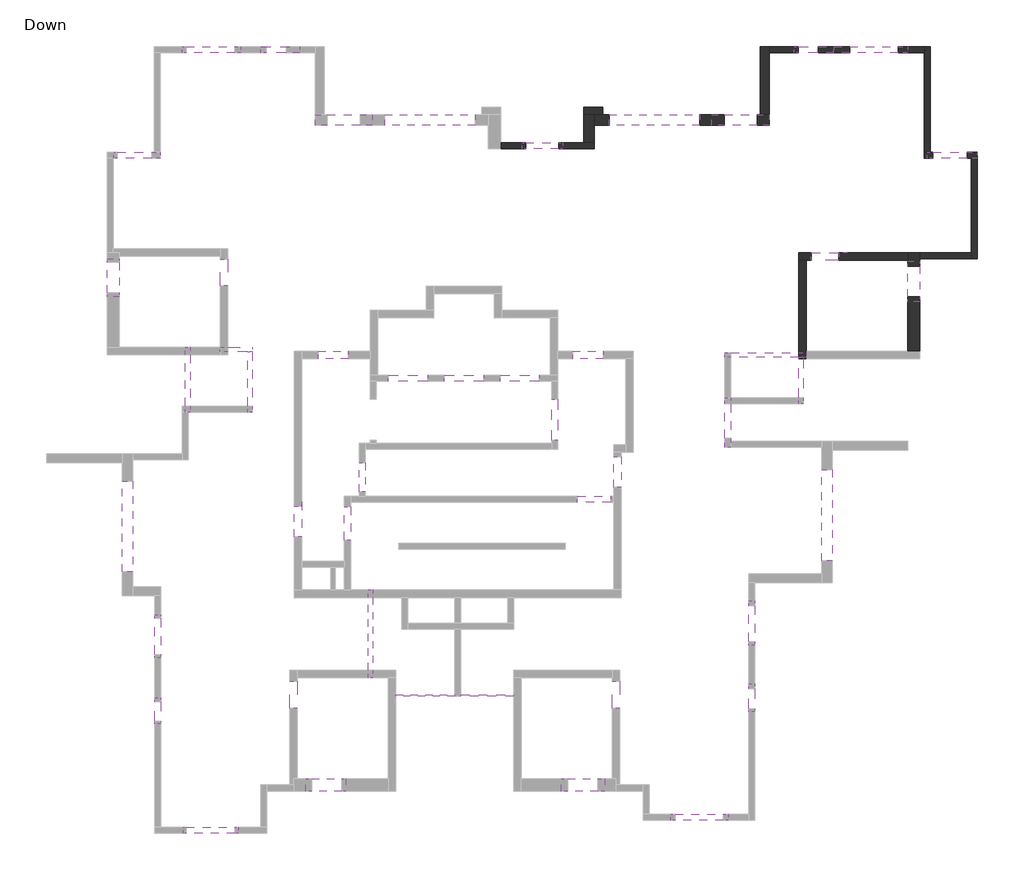
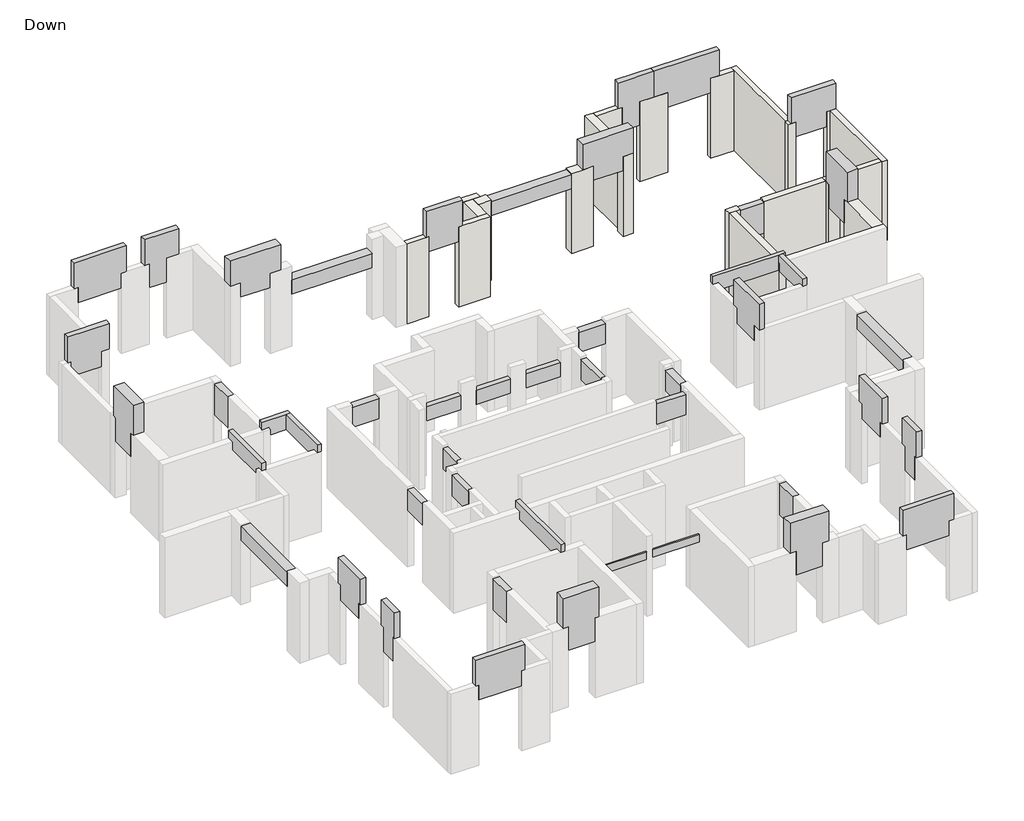
# One storey, part 3 of 3: 47 beams, 21 walls.
"""IFC4 building model written with IfcOpenShell, lengths in millimetres."""

from ifc_helpers import new_model, si_unit, frame, origin, place, context, project, spatial, polyline, outline, extrude, faceted_brep, element, save

model = new_model("IFC4")

# Units and contexts
model_context = context("Model", 3, world=origin())
ifc_project = project(units=[si_unit("LENGTHUNIT", "METRE", prefix="MILLI")], contexts=[model_context])

# Site, building, storey
site = spatial("IfcSite", under=ifc_project)
building = spatial("IfcBuilding", under=site)
storey = spatial("IfcBuildingStorey", under=building, Name="Down", Elevation=0.0)

# Beams
placement = place(None, origin())
element("IfcBeam", 1, ObjectType="Concrete Rectengular Beam : 15/60", at=placement, inside=storey, context=model_context, shape_type="Brep", body=[
    faceted_brep([(-3745.4992849, -160.4554551, 3450.0), (-3745.4992849, -10.4554551, 3450.0), (-6449.3881109, -10.4554551, 3450.0), (-6449.3881109, -160.4554551, 3450.0), (-3995.4992849, -160.4554551, 3450.0), (-3845.4992849, -160.4554551, 3450.0), (-6449.3881109, -160.4554551, 3150.0), (-6249.3881109, -160.4554551, 3150.0), (-6249.3881109, -160.4554551, 2850.0), (-3995.4992849, -160.4554551, 2850.0), (-3995.4992849, -160.4554551, 3150.0), (-3845.4992849, -160.4554551, 3150.0), (-3745.4992849, -160.4554551, 3150.0), (-3995.4992849, -10.4554551, 2850.0), (-6249.3881109, -10.4554551, 2850.0), (-3745.4992849, -10.4554551, 3150.0), (-3995.4992849, -10.4554551, 3150.0), (-3995.4992849, -10.4554551, 2950.0), (-6249.3881109, -10.4554551, 3150.0), (-6449.3881109, -10.4554551, 3150.0)], [[[0, 1, 2, 3, 4, 5]], [[0, 5, 4, 3, 6, 7, 8, 9, 10, 11, 12]], [[13, 9, 8, 14]], [[2, 1, 15, 16, 17, 13, 14, 18, 19]], [[1, 0, 12, 15]], [[3, 2, 19, 6]], [[16, 10, 9, 13, 17]], [[10, 16, 15, 12, 11]], [[7, 18, 14, 8]], [[18, 7, 6, 19]]]),
])
element("IfcBeam", 2, ObjectType="Concrete Rectengular Beam : 15/60", at=placement, inside=storey, context=model_context, shape_type="SweptSolid", body=[
    extrude(outline(polyline([(-1713.3876412, 3450.0), (-160.4554551, 3450.0), (-160.4554551, 3150.0), (-210.9535871, 3150.0), (-210.9535871, 2850.0), (-1513.3876412, 2850.0), (-1513.3876412, 3150.0), (-1713.3876412, 3150.0), (-1713.3876412, 3450.0)])), frame((-3995.4992849, 0.0, 0.0), z_axis=(1.0, 0.0, 0.0), x_axis=(0.0, 1.0, 0.0)), (0.0, 0.0, 1.0), 150.0),
])
element("IfcBeam", 3, ObjectType="Concrete Rectengular Beam : 15/60", at=placement, inside=storey, context=model_context, shape_type="Brep", body=[
    faceted_brep([(-23152.2127458, 170.2815538, 3450.0), (-23152.2127458, 20.2815538, 3450.0), (-22250.9487358, 20.2815538, 3450.0), (-22100.9487358, 20.2815538, 3450.0), (-22100.9487358, 170.2815538, 3450.0), (-23152.2127458, 20.2815538, 3150.0), (-22902.2127458, 20.2815538, 3150.0), (-22902.2127458, 20.2815538, 2850.0), (-22250.9487358, 20.2815538, 2850.0), (-22100.9487358, 20.2815538, 2850.0), (-22100.9487358, 20.2815538, 2950.0), (-22100.9487358, 20.2815538, 3150.0), (-22100.9487358, 170.2815538, 2850.0), (-22902.2127458, 170.2815538, 2850.0), (-22100.9487358, 170.2815538, 3150.0), (-22100.9487358, 170.2815538, 2950.0), (-22902.2127458, 170.2815538, 2950.0), (-22902.2127458, 170.2815538, 3150.0), (-23152.2127458, 170.2815538, 3150.0)], [[[0, 1, 2, 3, 4]], [[3, 2, 1, 5, 6, 7, 8, 9, 10, 11]], [[12, 9, 8, 7, 13]], [[0, 4, 14, 15, 12, 13, 16, 17, 18]], [[1, 0, 18, 5]], [[4, 3, 11, 10, 9, 12, 15, 14]], [[6, 17, 16, 13, 7]], [[17, 6, 5, 18]]]),
])
element("IfcBeam", 4, ObjectType="Concrete Rectengular Beam : 15/60", at=placement, inside=storey, context=model_context, shape_type="Brep", body=[
    faceted_brep([(-22250.9487358, -1984.190313, 3450.0), (-22100.9487358, -1984.190313, 3450.0), (-22100.9487358, 20.2815538, 3450.0), (-22250.9487358, 20.2815538, 3450.0), (-22250.9487358, 20.2815538, 2850.0), (-22250.9487358, -1784.190313, 2850.0), (-22250.9487358, -1784.190313, 3150.0), (-22250.9487358, -1984.190313, 3150.0), (-22100.9487358, 20.2815538, 2850.0), (-22100.9487358, -1784.190313, 2850.0), (-22100.9487358, -1984.190313, 3150.0), (-22100.9487358, -1784.190313, 3150.0), (-22100.9487358, 20.2815538, 2950.0), (-22100.9487358, 20.2815538, 3150.0)], [[[0, 1, 2, 3]], [[3, 4, 5, 6, 7, 0]], [[4, 8, 9, 5]], [[2, 1, 10, 11, 9, 8, 12, 13]], [[1, 0, 7, 10]], [[3, 2, 13, 12, 8, 4]], [[11, 6, 5, 9]], [[6, 11, 10, 7]]]),
])
element("IfcBeam", 5, ObjectType="Concrete Rectengular Beam : 15/60", at=placement, inside=storey, context=model_context, shape_type="SweptSolid", body=[
    extrude(outline(polyline([(-1984.190313, 3450.0), (170.2815538, 3450.0), (170.2815538, 3150.0), (-79.7184462, 3150.0), (-79.7184462, 2850.0), (-1784.190313, 2850.0), (-1784.190313, 3150.0), (-1984.190313, 3150.0), (-1984.190313, 3450.0)])), frame((-24310.0622873, 0.0, 0.0), z_axis=(1.0, 0.0, 0.0), x_axis=(0.0, 1.0, 0.0)), (0.0, 0.0, 1.0), 150.0),
])
element("IfcBeam", 6, ObjectType="Concrete Rectengular Beam : 15/60", at=placement, inside=storey, context=model_context, shape_type="Brep", body=[
    faceted_brep([(-18253.1541021, -10778.5353827, 3450.0), (-18103.1541021, -10778.5353827, 3450.0), (-18103.1541021, -7874.1201217, 3450.0), (-18253.1541021, -7874.1201217, 3450.0), (-18103.1541021, -10778.5353827, 3150.0), (-18103.1541021, -10528.5353827, 3150.0), (-18103.1541021, -10528.5353827, 3000.0), (-18103.1541021, -10528.5353827, 2850.0), (-18103.1541021, -8124.1201217, 2850.0), (-18103.1541021, -8124.1201217, 3000.0), (-18103.1541021, -8124.1201217, 3150.0), (-18103.1541021, -7874.1201217, 3150.0), (-18253.1541021, -10528.5353827, 2850.0), (-18253.1541021, -8124.1201217, 2850.0), (-18253.1541021, -7874.1201217, 3150.0), (-18253.1541021, -8124.1201217, 3150.0), (-18253.1541021, -8124.1201217, 2950.0), (-18253.1541021, -10528.5353827, 2950.0), (-18253.1541021, -10528.5353827, 3150.0), (-18253.1541021, -10778.5353827, 3150.0)], [[[0, 1, 2, 3]], [[2, 1, 4, 5, 6, 7, 8, 9, 10, 11]], [[7, 12, 13, 8]], [[0, 3, 14, 15, 16, 13, 12, 17, 18, 19]], [[1, 0, 19, 4]], [[3, 2, 11, 14]], [[5, 18, 17, 12, 7, 6]], [[18, 5, 4, 19]], [[15, 10, 9, 8, 13, 16]], [[10, 15, 14, 11]]]),
])
element("IfcBeam", 7, ObjectType="Concrete Rectengular Beam : 20/160", at=placement, inside=storey, context=model_context, shape_type="SweptSolid", body=[
    extrude(outline(polyline([(4170.0, -25146.2068588), (4170.0, -26693.7048776), (3150.0, -26693.7048776), (3150.0, -26578.3590155), (2570.0, -26578.3590155), (2570.0, -25426.4061116), (3150.0, -25426.4061116), (3150.0, -25146.2068588), (4170.0, -25146.2068588)])), frame((0.0, 6420.0664514, 0.0), z_axis=(0.0, 1.0, 0.0), x_axis=(0.0, 0.0, 1.0)), (0.0, 0.0, 1.0), 200.0),
])
element("IfcBeam", 8, ObjectType="Concrete Rectengular Beam : 20/160", at=placement, inside=storey, context=model_context, shape_type="SweptSolid", body=[
    extrude(outline(polyline([(4170.0, -22484.8686951), (4170.0, -24424.8686951), (3150.0, -24424.8686951), (3150.0, -24284.8686951), (2570.0, -24284.8686951), (2570.0, -22681.9251878), (3150.0, -22681.9251878), (3150.0, -22484.8686951), (4170.0, -22484.8686951)])), frame((0.0, 9925.9195024, 0.0), z_axis=(0.0, 1.0, 0.0), x_axis=(0.0, 0.0, 1.0)), (0.0, 0.0, 1.0), 200.0),
])
element("IfcBeam", 9, ObjectType="Concrete Rectengular Beam : 20/160", at=placement, inside=storey, context=model_context, shape_type="SweptSolid", body=[
    extrude(outline(polyline([(4170.0, -11807.2982207), (4170.0, -13147.2982207), (3150.0, -13147.2982207), (3150.0, -13043.4331692), (2570.0, -13043.4331692), (2570.0, -11941.4746047), (3150.0, -11941.4746047), (3150.0, -11807.2982207), (4170.0, -11807.2982207)])), frame((0.0, 6745.5504319, 0.0), z_axis=(0.0, 1.0, 0.0), x_axis=(0.0, 0.0, 1.0)), (0.0, 0.0, 1.0), 200.0),
])
element("IfcBeam", 10, ObjectType="Concrete Rectengular Beam : 20/160", at=placement, inside=storey, context=model_context, shape_type="SweptSolid", body=[
    extrude(outline(polyline([(4170.0, -388.4439243), (4170.0, -2828.4439243), (3150.0, -2828.4439243), (3150.0, -2302.4618118), (2570.0, -2302.4618118), (2570.0, -700.0390789), (3150.0, -700.0390789), (3150.0, -388.4439243), (4170.0, -388.4439243)])), frame((0.0, 9926.4176344, 0.0), z_axis=(0.0, 1.0, 0.0), x_axis=(0.0, 0.0, 1.0)), (0.0, 0.0, 1.0), 200.0),
])
element("IfcBeam", 11, ObjectType="Concrete Rectengular Beam : 20/160", at=placement, inside=storey, context=model_context, shape_type="SweptSolid", body=[
    extrude(outline(polyline([(4170.0, 1924.6637401), (4170.0, 261.8198592), (3150.0, 261.8198592), (3150.0, 442.019112), (2570.0, 442.019112), (2570.0, 1593.9720159), (3150.0, 1593.9720159), (3150.0, 1924.6637401), (4170.0, 1924.6637401)])), frame((0.0, 6420.0664514, 0.0), z_axis=(0.0, 1.0, 0.0), x_axis=(0.0, 0.0, 1.0)), (0.0, 0.0, 1.0), 200.0),
])
element("IfcBeam", 12, ObjectType="Concrete Rectengular Beam : 20/160", at=placement, inside=storey, context=model_context, shape_type="SweptSolid", body=[
    extrude(outline(polyline([(-3145.5397979, 4170.0), (-1513.3876412, 4170.0), (-1513.3876412, 3150.0), (-1713.3876412, 3150.0), (-1713.3876412, 2570.0), (-2845.5511191, 2570.0), (-2845.5511191, 3150.0), (-3145.5397979, 3150.0), (-3145.5397979, 4170.0)])), frame((-6449.3881109, 0.0, 0.0), z_axis=(1.0, 0.0, 0.0), x_axis=(0.0, 1.0, 0.0)), (0.0, 0.0, 1.0), 200.0),
])
element("IfcBeam", 13, ObjectType="Concrete Rectengular Beam : 20/160", at=placement, inside=storey, context=model_context, shape_type="SweptSolid", body=[
    extrude(outline(polyline([(-9711.6622931, 4170.0), (-8231.6622931, 4170.0), (-8231.6622931, 3150.0), (-8389.7150498, 3150.0), (-8389.7150498, 2570.0), (-9591.6622931, 2570.0), (-9591.6622931, 3150.0), (-9711.6622931, 3150.0), (-9711.6622931, 4170.0)])), frame((-5648.4371316, 0.0, 0.0), z_axis=(1.0, 0.0, 0.0), x_axis=(0.0, 1.0, 0.0)), (0.0, 0.0, 1.0), 200.0),
])
element("IfcBeam", 14, ObjectType="Concrete Rectengular Beam : 20/160", at=placement, inside=storey, context=model_context, shape_type="SweptSolid", body=[
    extrude(outline(polyline([(4170.0, -6333.7920507), (4170.0, -8233.7920507), (3150.0, -8233.7920507), (3150.0, -8093.7920507), (2570.0, -8093.7920507), (2570.0, -6499.9032247), (3150.0, -6499.9032247), (3150.0, -6333.7920507), (4170.0, -6333.7920507)])), frame((0.0, -15507.4032645, 0.0), z_axis=(0.0, 1.0, 0.0), x_axis=(0.0, 0.0, 1.0)), (0.0, 0.0, 1.0), 200.0),
])
element("IfcBeam", 15, ObjectType="Concrete Rectengular Beam : 20/160", at=placement, inside=storey, context=model_context, shape_type="SweptSolid", body=[
    extrude(outline(polyline([(4170.0, -22565.2739934), (4170.0, -24385.2739934), (3150.0, -24385.2739934), (3150.0, -24279.6609514), (2570.0, -24279.6609514), (2570.0, -22676.7174441), (3150.0, -22676.7174441), (3150.0, -22565.2739934), (4170.0, -22565.2739934)])), frame((0.0, -15927.4032645, 0.0), z_axis=(0.0, 1.0, 0.0), x_axis=(0.0, 0.0, 1.0)), (0.0, 0.0, 1.0), 200.0),
])
element("IfcBeam", 16, ObjectType="Concrete Rectengular Beam : 20/160", at=placement, inside=storey, context=model_context, shape_type="SweptSolid", body=[
    extrude(outline(polyline([(-10112.4479831, 4170.0), (-8692.4479831, 4170.0), (-8692.4479831, 3150.0), (-8810.5007399, 3150.0), (-8810.5007399, 2570.0), (-10012.4479831, 2570.0), (-10012.4479831, 3150.0), (-10112.4479831, 3150.0), (-10112.4479831, 4170.0)])), frame((-25331.1270445, 0.0, 0.0), z_axis=(1.0, 0.0, 0.0), x_axis=(0.0, 1.0, 0.0)), (0.0, 0.0, 1.0), 200.0),
])
element("IfcBeam", 17, ObjectType="Concrete Rectengular Beam : 20/195", at=placement, inside=storey, context=model_context, shape_type="Brep", body=[
    faceted_brep([(-20529.9609627, 10126.4176344, 4170.0), (-20529.9609627, 9926.4176344, 4170.0), (-20529.9609627, 9926.4176344, 3150.0), (-20529.9609627, 10125.9195024, 3150.0), (-20529.9609627, 10125.9195024, 2220.0), (-20529.9609627, 10126.4176344, 2220.0), (-21809.9609627, 10126.4176344, 4170.0), (-21809.9609627, 10126.4176344, 2220.0), (-21809.9609627, 10125.9195024, 2220.0), (-21809.9609627, 10125.9195024, 3150.0), (-21809.9609627, 9926.4176344, 3150.0), (-21809.9609627, 9926.4176344, 4170.0), (-21629.9609627, 9926.4176344, 3150.0), (-21629.9609627, 9926.4176344, 2220.0), (-20978.9930017, 9926.4176344, 2220.0), (-20978.9930017, 9926.4176344, 3150.0), (-20978.9930017, 10125.9195024, 2220.0), (-21629.9609627, 10125.9195024, 2220.0), (-21629.9609627, 10125.9195024, 3150.0), (-20978.9930017, 10125.9195024, 3150.0)], [[[0, 1, 2, 3, 4, 5]], [[6, 7, 8, 9, 10, 11]], [[1, 0, 6, 11]], [[1, 11, 10, 12, 13, 14, 15, 2]], [[7, 5, 4, 16, 14, 13, 17, 8]], [[0, 5, 7, 6]], [[17, 18, 9, 8]], [[18, 17, 13, 12]], [[9, 18, 12, 10]], [[3, 19, 16, 4]], [[19, 3, 2, 15]], [[16, 19, 15, 14]]]),
])
element("IfcBeam", 18, ObjectType="Concrete Rectengular Beam : 20/195", at=placement, inside=storey, context=model_context, shape_type="SweptSolid", body=[
    extrude(outline(polyline([(4170.0, -2828.4439243), (4170.0, -4145.3939979), (3150.0, -4145.3939979), (3150.0, -4005.3939979), (2220.0, -4005.3939979), (2220.0, -3354.4260369), (3150.0, -3354.4260369), (3150.0, -2828.4439243), (4170.0, -2828.4439243)])), frame((0.0, 9926.4176344, 0.0), z_axis=(0.0, 1.0, 0.0), x_axis=(0.0, 0.0, 1.0)), (0.0, 0.0, 1.0), 200.0),
])
element("IfcBeam", 19, ObjectType="Concrete Rectengular Beam : 20/195", at=placement, inside=storey, context=model_context, shape_type="SweptSolid", body=[
    extrude(outline(polyline([(-11906.6175745, 4170.0), (-10986.6175745, 4170.0), (-10986.6175745, 3150.0), (-11149.2984303, 3150.0), (-11149.2984303, 2220.0), (-11806.6175745, 2220.0), (-11806.6175745, 3150.0), (-11906.6175745, 3150.0), (-11906.6175745, 4170.0)])), frame((-5648.4371316, 0.0, 0.0), z_axis=(1.0, 0.0, 0.0), x_axis=(0.0, 1.0, 0.0)), (0.0, 0.0, 1.0), 200.0),
])
element("IfcBeam", 20, ObjectType="Concrete Rectengular Beam : 20/195", at=placement, inside=storey, context=model_context, shape_type="SweptSolid", body=[
    extrude(outline(polyline([(-12301.0520814, 4170.0), (-11441.0520814, 4170.0), (-11441.0520814, 3150.0), (-11570.0841204, 3150.0), (-11570.0841204, 2220.0), (-12221.0520814, 2220.0), (-12221.0520814, 3150.0), (-12301.0520814, 3150.0), (-12301.0520814, 4170.0)])), frame((-25331.1270445, 0.0, 0.0), z_axis=(1.0, 0.0, 0.0), x_axis=(0.0, 1.0, 0.0)), (0.0, 0.0, 1.0), 200.0),
])
element("IfcBeam", 21, ObjectType="Concrete Rectengular Beam : 20/55", at=placement, inside=storey, context=model_context, shape_type="SweptSolid", body=[
    extrude(outline(polyline([(-16290.9821333, -762.4310014), (-16290.9821333, -962.4310014), (-17593.4388298, -962.4310014), (-17593.4388298, -762.4310014), (-16290.9821333, -762.4310014)])), frame((0.0, 0.0, 2150.0), z_axis=(0.0, 0.0, 1.0), x_axis=(1.0, 0.0, 0.0)), (0.0, 0.0, 1.0), 550.0),
])
element("IfcBeam", 22, ObjectType="Concrete Rectengular Beam : 20/55", at=placement, inside=storey, context=model_context, shape_type="SweptSolid", body=[
    extrude(outline(polyline([(-14438.066929, -762.4310014), (-14438.066929, -962.4310014), (-15740.0028511, -962.4310014), (-15740.0028511, -762.4310014), (-14438.066929, -762.4310014)])), frame((0.0, 0.0, 2150.0), z_axis=(0.0, 0.0, 1.0), x_axis=(1.0, 0.0, 0.0)), (0.0, 0.0, 1.0), 550.0),
])
element("IfcBeam", 23, ObjectType="Concrete Rectengular Beam : 20/55", at=placement, inside=storey, context=model_context, shape_type="SweptSolid", body=[
    extrude(outline(polyline([(-12584.1498, -762.4310014), (-12584.1498, -962.4310014), (-13887.0876467, -962.4310014), (-13887.0876467, -762.4310014), (-12584.1498, -762.4310014)])), frame((0.0, 0.0, 2150.0), z_axis=(0.0, 0.0, 1.0), x_axis=(1.0, 0.0, 0.0)), (0.0, 0.0, 1.0), 550.0),
])
element("IfcBeam", 24, ObjectType="Concrete Rectengular Beam : 20/80", at=placement, inside=storey, context=model_context, shape_type="SweptSolid", body=[
    extrude(outline(polyline([(-18550.1013454, -3666.8122988), (-18350.1013454, -3666.8122988), (-18350.1013454, -4618.2670707), (-18550.1013454, -4618.2670707), (-18550.1013454, -3666.8122988)])), frame((0.0, 0.0, 2250.0), z_axis=(0.0, 0.0, 1.0), x_axis=(1.0, 0.0, 0.0)), (0.0, 0.0, 1.0), 800.0),
])
element("IfcBeam", 25, ObjectType="Concrete Rectengular Beam : 20/80", at=placement, inside=storey, context=model_context, shape_type="SweptSolid", body=[
    extrude(outline(polyline([(-10226.0438338, -4768.7708633), (-10226.0438338, -4968.7708633), (-11328.0023982, -4968.7708633), (-11328.0023982, -4768.7708633), (-10226.0438338, -4768.7708633)])), frame((0.0, 0.0, 2250.0), z_axis=(0.0, 0.0, 1.0), x_axis=(1.0, 0.0, 0.0)), (0.0, 0.0, 1.0), 800.0),
])
element("IfcBeam", 26, ObjectType="Concrete Rectengular Beam : 20/80", at=placement, inside=storey, context=model_context, shape_type="SweptSolid", body=[
    extrude(outline(polyline([(-12184.178103, -1563.404623), (-11984.178103, -1563.404623), (-11984.178103, -2915.3348845), (-12184.178103, -2915.3348845), (-12184.178103, -1563.404623)])), frame((0.0, 0.0, 2250.0), z_axis=(0.0, 0.0, 1.0), x_axis=(1.0, 0.0, 0.0)), (0.0, 0.0, 1.0), 800.0),
])
element("IfcBeam", 27, ObjectType="Concrete Rectengular Beam : 20/80", at=placement, inside=storey, context=model_context, shape_type="SweptSolid", body=[
    extrude(outline(polyline([(3050.0, -18848.2746727), (3050.0, -19043.2746727), (2250.0, -19043.2746727), (2250.0, -18843.2746727), (2950.0, -18843.2746727), (2950.0, -18848.2746727), (3050.0, -18848.2746727)])), frame((0.0, -6221.210578, 0.0), z_axis=(0.0, 1.0, 0.0), x_axis=(0.0, 0.0, 1.0)), (0.0, 0.0, 1.0), 1101.9585645),
])
element("IfcBeam", 28, ObjectType="Concrete Rectengular Beam : 25/120", at=placement, inside=storey, context=model_context, shape_type="SweptSolid", body=[
    extrude(outline(polyline([(-23152.2127458, 3085.0930561), (-22902.2127458, 3085.0930561), (-22902.2127458, 2208.0433561), (-23152.2127458, 2208.0433561), (-23152.2127458, 3085.0930561)])), frame((0.0, 0.0, 1900.0), z_axis=(0.0, 0.0, 1.0), x_axis=(1.0, 0.0, 0.0)), (0.0, 0.0, 1.0), 1200.0),
])
element("IfcBeam", 29, ObjectType="Concrete Rectengular Beam : 25/120", at=placement, inside=storey, context=model_context, shape_type="Brep", body=[
    faceted_brep([(-2382.6064399, 3294.8994639, 1900.0), (-2382.6064399, 3294.8994639, 2950.0), (-2382.6064399, 3294.4013319, 2950.0), (-2382.6064399, 3294.4013319, 1900.0), (-2675.3362599, 3044.8994639, 3100.0), (-2675.3362599, 3294.4013319, 3100.0), (-3574.7135949, 3294.4013319, 3100.0), (-3574.7135949, 3044.8994639, 3100.0), (-2675.3362599, 3044.8994639, 1900.0), (-2675.3362599, 3044.8994639, 2860.0), (-3574.7135949, 3044.8994639, 1900.0), (-2675.3362599, 3294.4013319, 1900.0), (-3574.7135949, 3294.8994639, 1900.0), (-3574.7135949, 3294.8994639, 2950.0), (-3574.7135949, 3294.4013319, 2950.0), (-2675.3362599, 3294.4013319, 2950.0)], [[[0, 1, 2, 3]], [[4, 5, 6, 7]], [[8, 9, 4, 7, 10]], [[0, 3, 11, 8, 10, 12]], [[1, 0, 12, 13]], [[2, 1, 13, 14, 15]], [[5, 15, 14, 6]], [[15, 11, 3, 2]], [[11, 15, 5, 4, 9, 8]], [[7, 6, 14, 13, 12, 10]]]),
])
element("IfcBeam", 30, ObjectType="Concrete Rectengular Beam : 25/120", at=placement, inside=storey, context=model_context, shape_type="SweptSolid", body=[
    extrude(outline(polyline([(-9925.0588909, -11794.8752446), (-10175.0588909, -11794.8752446), (-10175.0588909, -10898.8059589), (-9925.0588909, -10898.8059589), (-9925.0588909, -11794.8752446)])), frame((0.0, 0.0, 1900.0), z_axis=(0.0, 0.0, 1.0), x_axis=(1.0, 0.0, 0.0)), (0.0, 0.0, 1.0), 1200.0),
])
element("IfcBeam", 31, ObjectType="Concrete Rectengular Beam : 25/120", at=placement, inside=storey, context=model_context, shape_type="SweptSolid", body=[
    extrude(outline(polyline([(-20604.0071531, -11794.8752446), (-20854.0071531, -11794.8752446), (-20854.0071531, -10898.8059589), (-20604.0071531, -10898.8059589), (-20604.0071531, -11794.8752446)])), frame((0.0, 0.0, 1900.0), z_axis=(0.0, 0.0, 1.0), x_axis=(1.0, 0.0, 0.0)), (0.0, 0.0, 1.0), 1200.0),
])
element("IfcBeam", 32, ObjectType="Concrete Rectengular Beam : 25/80", at=placement, inside=storey, context=model_context, shape_type="SweptSolid", body=[
    extrude(outline(polyline([(-19917.1340636, -210.4611157), (-19917.1340636, 39.5388843), (-18915.6849523, 39.5388843), (-18915.6849523, -210.4611157), (-19917.1340636, -210.4611157)])), frame((0.0, 0.0, 2250.0), z_axis=(0.0, 0.0, 1.0), x_axis=(1.0, 0.0, 0.0)), (0.0, 0.0, 1.0), 800.0),
])
element("IfcBeam", 33, ObjectType="Concrete Rectengular Beam : 25/80", at=placement, inside=storey, context=model_context, shape_type="SweptSolid", body=[
    extrude(outline(polyline([(-11477.9854165, -210.9535871), (-11477.9854165, 39.0464129), (-10476.5363052, 39.0464129), (-10476.5363052, -210.9535871), (-11477.9854165, -210.9535871)])), frame((0.0, 0.0, 2250.0), z_axis=(0.0, 0.0, 1.0), x_axis=(1.0, 0.0, 0.0)), (0.0, 0.0, 1.0), 800.0),
])
element("IfcBeam", 34, ObjectType="Concrete Rectengular Beam : 25/80", at=placement, inside=storey, context=model_context, shape_type="SweptSolid", body=[
    extrude(outline(polyline([(-9876.055155, -4468.2840524), (-10126.055155, -4468.2840524), (-10126.055155, -3466.3141668), (-9876.055155, -3466.3141668), (-9876.055155, -4468.2840524)])), frame((0.0, 0.0, 2250.0), z_axis=(0.0, 0.0, 1.0), x_axis=(1.0, 0.0, 0.0)), (0.0, 0.0, 1.0), 800.0),
])
element("IfcBeam", 35, ObjectType="Concrete Rectengular Beam : 25/80", at=placement, inside=storey, context=model_context, shape_type="Brep", body=[
    faceted_brep([(-20453.0108891, -4948.7708633, 2950.0), (-20453.0108891, -4948.7708633, 2250.0), (-20453.5033605, -4948.7708633, 2250.0), (-20453.5033605, -4948.7708633, 2950.0), (-20703.0108891, -6110.8064118, 3050.0), (-20453.5033605, -6110.8064118, 3050.0), (-20453.5033605, -5109.3573005, 3050.0), (-20703.0108891, -5109.3573005, 3050.0), (-20453.0108891, -6110.8064118, 2950.0), (-20453.0108891, -6110.8064118, 2250.0), (-20703.0108891, -6110.8064118, 2250.0), (-20703.0108891, -5109.3573005, 2250.0), (-20453.5033605, -5109.3573005, 2250.0), (-20703.0108891, -5109.3573005, 2950.0), (-20453.5033605, -5109.3573005, 2950.0), (-20453.5033605, -6110.8064118, 2950.0)], [[[0, 1, 2, 3]], [[4, 5, 6, 7]], [[1, 0, 8, 9]], [[1, 9, 10, 11, 12, 2]], [[10, 4, 7, 13, 11]], [[0, 3, 14, 15, 8]], [[5, 15, 14, 6]], [[5, 4, 10, 9, 8, 15]], [[12, 14, 3, 2]], [[14, 12, 11, 13, 7, 6]]]),
])
element("IfcBeam", 36, ObjectType="Concrete Rectengular Beam : 35/155", at=placement, inside=storey, context=model_context, shape_type="SweptSolid", body=[
    extrude(outline(polyline([(4150.0, -18115.5151346), (4150.0, -20006.7412186), (3150.0, -20006.7412186), (3150.0, -19621.8549965), (2600.0, -19621.8549965), (2600.0, -18519.896432), (3150.0, -18519.896432), (3150.0, -18115.5151346), (4150.0, -18115.5151346)])), frame((0.0, 7522.5061661, 0.0), z_axis=(0.0, 1.0, 0.0), x_axis=(0.0, 0.0, 1.0)), (0.0, 0.0, 1.0), 350.0),
])
element("IfcBeam", 37, ObjectType="Concrete Rectengular Beam : 35/155", at=placement, inside=storey, context=model_context, shape_type="SweptSolid", body=[
    extrude(outline(polyline([(4150.0, -4977.1589702), (4150.0, -6868.871865), (3150.0, -6868.871865), (3150.0, -6464.4905676), (2600.0, -6464.4905676), (2600.0, -5362.5320031), (3150.0, -5362.5320031), (3150.0, -4977.1589702), (4150.0, -4977.1589702)])), frame((0.0, 7522.0250158, 0.0), z_axis=(0.0, 1.0, 0.0), x_axis=(0.0, 0.0, 1.0)), (0.0, 0.0, 1.0), 350.0),
])
element("IfcBeam", 38, ObjectType="Concrete Rectengular Beam : 35/50", at=placement, inside=storey, context=model_context, shape_type="SweptSolid", body=[
    extrude(outline(polyline([(-10278.642045, 7522.0250158), (-10278.642045, 7872.0250158), (-7273.2531624, 7872.0250158), (-7273.2531624, 7522.0250158), (-10278.642045, 7522.0250158)])), frame((0.0, 0.0, 2550.0), z_axis=(0.0, 0.0, 1.0), x_axis=(1.0, 0.0, 0.0)), (0.0, 0.0, 1.0), 550.0),
])
element("IfcBeam", 39, ObjectType="Concrete Rectengular Beam : 35/50", at=placement, inside=storey, context=model_context, shape_type="SweptSolid", body=[
    extrude(outline(polyline([(-2887.9389996, -6903.0129016), (-3237.9389996, -6903.0129016), (-3237.9389996, -3892.3076005), (-2887.9389996, -3892.3076005), (-2887.9389996, -6903.0129016)])), frame((0.0, 0.0, 2550.0), z_axis=(0.0, 0.0, 1.0), x_axis=(1.0, 0.0, 0.0)), (0.0, 0.0, 1.0), 550.0),
])
element("IfcBeam", 40, ObjectType="Concrete Rectengular Beam : 35/50", at=placement, inside=storey, context=model_context, shape_type="SweptSolid", body=[
    extrude(outline(polyline([(-26412.7923903, -4267.7859204), (-26062.7923903, -4267.7859204), (-26062.7923903, -7272.6540287), (-26412.7923903, -7272.6540287), (-26412.7923903, -4267.7859204)])), frame((0.0, 0.0, 2550.0), z_axis=(0.0, 0.0, 1.0), x_axis=(1.0, 0.0, 0.0)), (0.0, 0.0, 1.0), 550.0),
])
element("IfcBeam", 41, ObjectType="Concrete Rectengular Beam : 35/55", at=placement, inside=storey, context=model_context, shape_type="SweptSolid", body=[
    extrude(outline(polyline([(-14706.2657289, 7872.5061661), (-14706.2657289, 7522.5061661), (-17711.1338372, 7522.5061661), (-17711.1338372, 7872.5061661), (-14706.2657289, 7872.5061661)])), frame((0.0, 0.0, 2050.0), z_axis=(0.0, 0.0, 1.0), x_axis=(1.0, 0.0, 0.0)), (0.0, 0.0, 1.0), 550.0),
])
element("IfcBeam", 42, ObjectType="Concrete Rectengular Beam : 40/210", at=placement, inside=storey, context=model_context, shape_type="SweptSolid", body=[
    extrude(outline(polyline([(1674.4013319, 4330.0), (3019.1550962, 4330.0), (3019.1550962, 3150.0), (2843.9088605, 3150.0), (2843.9088605, 2230.0), (1842.4597492, 2230.0), (1842.4597492, 3150.0), (1674.4013319, 3150.0), (1674.4013319, 4330.0)])), frame((-388.661291, 0.0, 0.0), z_axis=(1.0, 0.0, 0.0), x_axis=(0.0, 1.0, 0.0)), (0.0, 0.0, 1.0), 400.0),
])
element("IfcBeam", 43, ObjectType="Concrete Rectengular Beam : 40/210", at=placement, inside=storey, context=model_context, shape_type="SweptSolid", body=[
    extrude(outline(polyline([(1832.6533414, 4330.0), (3092.6533414, 4330.0), (3092.6533414, 3150.0), (2974.1024527, 3150.0), (2974.1024527, 2230.0), (1972.6533414, 2230.0), (1972.6533414, 3150.0), (1832.6533414, 3150.0), (1832.6533414, 4330.0)])), frame((-26909.0507397, 0.0, 0.0), z_axis=(1.0, 0.0, 0.0), x_axis=(0.0, 1.0, 0.0)), (0.0, 0.0, 1.0), 400.0),
])
element("IfcBeam", 44, ObjectType="Concrete Rectengular Beam : 40/210", at=placement, inside=storey, context=model_context, shape_type="SweptSolid", body=[
    extrude(outline(polyline([(4330.0, -18998.1541021), (4330.0, -20318.1541021), (3150.0, -20318.1541021), (3150.0, -20132.7346523), (2230.0, -20132.7346523), (2230.0, -19133.1541021), (3150.0, -19133.1541021), (3150.0, -18998.1541021), (4330.0, -18998.1541021)])), frame((0.0, -14534.8752446, 0.0), z_axis=(0.0, 1.0, 0.0), x_axis=(0.0, 0.0, 1.0)), (0.0, 0.0, 1.0), 400.0),
])
element("IfcBeam", 45, ObjectType="Concrete Rectengular Beam : 40/210", at=placement, inside=storey, context=model_context, shape_type="SweptSolid", body=[
    extrude(outline(polyline([(4330.0, -10427.4710574), (4330.0, -11867.4710574), (3150.0, -11867.4710574), (3150.0, -11647.4710574), (2230.0, -11647.4710574), (2230.0, -10646.8295238), (3150.0, -10646.8295238), (3150.0, -10427.4710574), (4330.0, -10427.4710574)])), frame((0.0, -14534.8752446, 0.0), z_axis=(0.0, 1.0, 0.0), x_axis=(0.0, 0.0, 1.0)), (0.0, 0.0, 1.0), 400.0),
])
element("IfcBeam", 46, ObjectType="Concrete Rectengular Beam : 5/30", at=placement, inside=storey, context=model_context, shape_type="SweptSolid", body=[
    extrude(outline(polyline([(-17348.1541021, -11388.1261219), (-17348.1541021, -11338.1261219), (-15389.5217009, -11338.1261219), (-15389.5217009, -11388.1261219), (-17348.1541021, -11388.1261219)])), frame((0.0, 0.0, 2250.0), z_axis=(0.0, 0.0, 1.0), x_axis=(1.0, 0.0, 0.0)), (0.0, 0.0, 1.0), 300.0),
])
element("IfcBeam", 47, ObjectType="Concrete Rectengular Beam : 5/30", at=placement, inside=storey, context=model_context, shape_type="SweptSolid", body=[
    extrude(outline(polyline([(-15189.5217009, -11388.1261219), (-15189.5217009, -11338.1261219), (-13430.911942, -11338.1261219), (-13430.911942, -11388.1261219), (-15189.5217009, -11388.1261219)])), frame((0.0, 0.0, 2250.0), z_axis=(0.0, 0.0, 1.0), x_axis=(1.0, 0.0, 0.0)), (0.0, 0.0, 1.0), 300.0),
])

# Walls
element("IfcWall", 48, ObjectType="20", at=placement, inside=storey, context=model_context, shape_type="Brep", body=[
    faceted_brep([(-13867.2982207, 6745.5504319, 0.0), (-13043.4331692, 6745.5504319, 0.0), (-13043.4331692, 6745.5504319, 2570.0), (-13043.4331692, 6745.5504319, 3150.0), (-13147.2982207, 6745.5504319, 3150.0), (-13867.2982207, 6745.5504319, 3150.0), (-13867.2982207, 6945.5504319, 0.0), (-13867.2982207, 6945.5504319, 3150.0), (-13147.2982207, 6945.5504319, 3150.0), (-13043.4331692, 6945.5504319, 3150.0), (-13043.4331692, 6945.5504319, 2570.0), (-13043.4331692, 6945.5504319, 0.0)], [[[0, 1, 2, 3, 4, 5]], [[6, 7, 8, 9, 10, 11]], [[1, 0, 6, 11]], [[3, 2, 1, 11, 10, 9]], [[5, 4, 3, 9, 8, 7]], [[0, 5, 7, 6]]]),
])
element("IfcWall", 49, ObjectType="20", at=placement, inside=storey, context=model_context, shape_type="Brep", body=[
    faceted_brep([(-4977.1589702, 9926.4176344, 0.0), (-4005.3939979, 9926.4176344, 0.0), (-4005.3939979, 9926.4176344, 2220.0), (-4005.3939979, 9926.4176344, 3150.0), (-4145.3939979, 9926.4176344, 3150.0), (-4977.1589702, 9926.4176344, 3150.0), (-4977.1589702, 9926.4176344, 2950.0), (-4977.1589702, 10126.4176344, 0.0), (-4977.1589702, 10126.4176344, 3150.0), (-4145.3939979, 10126.4176344, 3150.0), (-4005.3939979, 10126.4176344, 3150.0), (-4005.3939979, 10126.4176344, 2220.0), (-4005.3939979, 10126.4176344, 0.0)], [[[0, 1, 2, 3, 4, 5, 6]], [[7, 8, 9, 10, 11, 12]], [[1, 0, 7, 12]], [[3, 2, 1, 12, 11, 10]], [[5, 4, 3, 10, 9, 8]], [[0, 6, 5, 8, 7]]]),
])
element("IfcWall", 50, ObjectType="20", at=placement, inside=storey, context=model_context, shape_type="Brep", body=[
    faceted_brep([(161.8198592, 10126.4176344, 0.0), (161.8198592, 9926.4176344, 0.0), (161.8198592, 6620.0664514, 0.0), (161.8198592, 6620.0664514, 2950.0), (161.8198592, 6620.0664514, 3150.0), (161.8198592, 9926.4176344, 3150.0), (161.8198592, 10126.4176344, 3150.0), (361.8198592, 10126.4176344, 0.0), (361.8198592, 10126.4176344, 3150.0), (361.8198592, 6620.0664514, 3150.0), (361.8198592, 6620.0664514, 0.0)], [[[0, 1, 2, 3, 4, 5, 6]], [[7, 8, 9, 10]], [[2, 1, 0, 7, 10]], [[6, 5, 4, 9, 8]], [[0, 6, 8, 7]], [[4, 3, 2, 10, 9]]]),
])
element("IfcWall", 51, ObjectType="20", at=placement, inside=storey, context=model_context, shape_type="Brep", body=[
    faceted_brep([(1593.9720159, 6420.0664514, 0.0), (1724.6637401, 6420.0664514, 0.0), (1924.6637401, 6420.0664514, 0.0), (1924.6637401, 6420.0664514, 3150.0), (1724.6637401, 6420.0664514, 3150.0), (1593.9720159, 6420.0664514, 3150.0), (1593.9720159, 6420.0664514, 2570.0), (1593.9720159, 6620.0664514, 0.0), (1593.9720159, 6620.0664514, 2570.0), (1593.9720159, 6620.0664514, 3150.0), (1924.6637401, 6620.0664514, 3150.0), (1924.6637401, 6620.0664514, 0.0)], [[[0, 1, 2, 3, 4, 5, 6]], [[7, 8, 9, 10, 11]], [[2, 1, 0, 7, 11]], [[5, 4, 3, 10, 9]], [[0, 6, 5, 9, 8, 7]], [[3, 2, 11, 10]]]),
])
element("IfcWall", 52, ObjectType="20", at=placement, inside=storey, context=model_context, shape_type="Brep", body=[
    faceted_brep([(1724.6637401, 6420.0664514, 0.0), (1724.6637401, 3294.4013319, 0.0), (1724.6637401, 3094.4013319, 0.0), (1724.6637401, 3094.4013319, 3150.0), (1724.6637401, 3294.4013319, 3150.0), (1724.6637401, 6420.0664514, 3150.0), (1724.6637401, 6420.0664514, 2950.0), (1924.6637401, 6420.0664514, 0.0), (1924.6637401, 6420.0664514, 3150.0), (1924.6637401, 3094.4013319, 3150.0), (1924.6637401, 3094.4013319, 0.0)], [[[0, 1, 2, 3, 4, 5, 6]], [[7, 8, 9, 10]], [[2, 1, 0, 7, 10]], [[5, 4, 3, 9, 8]], [[0, 6, 5, 8, 7]], [[3, 2, 10, 9]]]),
])
element("IfcWall", 53, ObjectType="20", at=placement, inside=storey, context=model_context, shape_type="Brep", body=[
    faceted_brep([(1724.6637401, 3294.4013319, 0.0), (11.338709, 3294.4013319, 0.0), (11.338709, 3294.4013319, 3150.0), (1724.6637401, 3294.4013319, 3150.0), (1724.6637401, 3294.4013319, 2950.0), (1724.6637401, 3094.4013319, 0.0), (1724.6637401, 3094.4013319, 3150.0), (11.338709, 3094.4013319, 3150.0), (11.338709, 3094.4013319, 0.0)], [[[0, 1, 2, 3, 4]], [[5, 6, 7, 8]], [[1, 0, 5, 8]], [[3, 2, 7, 6]], [[0, 4, 3, 6, 5]], [[2, 1, 8, 7]]]),
])
element("IfcWall", 54, ObjectType="20", at=placement, inside=storey, context=model_context, shape_type="Brep", body=[
    faceted_brep([(-11941.4746047, 6745.5504319, 0.0), (-10767.128403, 6745.5504319, 0.0), (-10767.128403, 6745.5504319, 2950.0), (-10767.128403, 6745.5504319, 3150.0), (-11807.2982207, 6745.5504319, 3150.0), (-11941.4746047, 6745.5504319, 3150.0), (-11941.4746047, 6745.5504319, 2570.0), (-11941.4746047, 6945.5504319, 0.0), (-11941.4746047, 6945.5504319, 2570.0), (-11941.4746047, 6945.5504319, 3150.0), (-11807.2982207, 6945.5504319, 3150.0), (-11117.6095532, 6945.5504319, 3150.0), (-10767.6095532, 6945.5504319, 3150.0), (-10767.128403, 6945.5504319, 3150.0), (-10767.128403, 6945.5504319, 2950.0), (-10767.128403, 6945.5504319, 0.0), (-10767.6095532, 6945.5504319, 0.0), (-11117.6095532, 6945.5504319, 0.0)], [[[0, 1, 2, 3, 4, 5, 6]], [[7, 8, 9, 10, 11, 12, 13, 14, 15, 16, 17]], [[1, 0, 7, 17, 16, 15]], [[3, 2, 1, 15, 14, 13]], [[5, 4, 3, 13, 12, 11, 10, 9]], [[0, 6, 5, 9, 8, 7]]]),
])
element("IfcWall", 55, ObjectType="20", at=placement, inside=storey, context=model_context, shape_type="Brep", body=[
    faceted_brep([(-3354.4260369, 9926.4176344, 0.0), (-2302.4618118, 9926.4176344, 0.0), (-2302.4618118, 9926.4176344, 2570.0), (-2302.4618118, 9926.4176344, 3150.0), (-2828.4439243, 9926.4176344, 3150.0), (-3354.4260369, 9926.4176344, 3150.0), (-3354.4260369, 9926.4176344, 2220.0), (-3354.4260369, 10126.4176344, 0.0), (-3354.4260369, 10126.4176344, 2220.0), (-3354.4260369, 10126.4176344, 3150.0), (-2828.4439243, 10126.4176344, 3150.0), (-2302.4618118, 10126.4176344, 3150.0), (-2302.4618118, 10126.4176344, 2570.0), (-2302.4618118, 10126.4176344, 0.0)], [[[0, 1, 2, 3, 4, 5, 6]], [[7, 8, 9, 10, 11, 12, 13]], [[1, 0, 7, 13]], [[3, 2, 1, 13, 12, 11]], [[5, 4, 3, 11, 10, 9]], [[0, 6, 5, 9, 8, 7]]]),
])
element("IfcWall", 56, ObjectType="20", at=placement, inside=storey, context=model_context, shape_type="Brep", body=[
    faceted_brep([(-700.0390789, 9926.4176344, 0.0), (161.8198592, 9926.4176344, 0.0), (161.8198592, 9926.4176344, 2950.0), (161.8198592, 9926.4176344, 3150.0), (-388.4439243, 9926.4176344, 3150.0), (-700.0390789, 9926.4176344, 3150.0), (-700.0390789, 9926.4176344, 2570.0), (-700.0390789, 10126.4176344, 0.0), (-700.0390789, 10126.4176344, 2570.0), (-700.0390789, 10126.4176344, 3150.0), (-388.4439243, 10126.4176344, 3150.0), (161.8198592, 10126.4176344, 3150.0), (161.8198592, 10126.4176344, 0.0)], [[[0, 1, 2, 3, 4, 5, 6]], [[7, 8, 9, 10, 11, 12]], [[1, 0, 7, 12]], [[5, 4, 3, 11, 10, 9]], [[0, 6, 5, 9, 8, 7]], [[3, 2, 1, 12, 11]]]),
])
element("IfcWall", 57, ObjectType="20", at=placement, inside=storey, context=model_context, shape_type="Brep", body=[
    faceted_brep([(161.3217272, 6420.0664514, 0.0), (442.019112, 6420.0664514, 0.0), (442.019112, 6420.0664514, 2570.0), (442.019112, 6420.0664514, 3150.0), (261.8198592, 6420.0664514, 3150.0), (161.3217272, 6420.0664514, 3150.0), (161.3217272, 6420.0664514, 2950.0), (161.3217272, 6620.0664514, 0.0), (161.3217272, 6620.0664514, 2950.0), (161.3217272, 6620.0664514, 3150.0), (161.8198592, 6620.0664514, 3150.0), (261.8198592, 6620.0664514, 3150.0), (361.8198592, 6620.0664514, 3150.0), (442.019112, 6620.0664514, 3150.0), (442.019112, 6620.0664514, 2570.0), (442.019112, 6620.0664514, 0.0), (361.8198592, 6620.0664514, 0.0), (161.8198592, 6620.0664514, 0.0)], [[[0, 1, 2, 3, 4, 5, 6]], [[7, 8, 9, 10, 11, 12, 13, 14, 15, 16, 17]], [[1, 0, 7, 17, 16, 15]], [[3, 2, 1, 15, 14, 13]], [[5, 4, 3, 13, 12, 11, 10, 9]], [[0, 6, 5, 9, 8, 7]]]),
])
element("IfcWall", 58, ObjectType="25", at=placement, inside=storey, context=model_context, shape_type="Brep", body=[
    faceted_brep([(-11117.6095532, 7872.0250158, 0.0), (-10767.6095532, 7872.0250158, 0.0), (-10489.03489, 7872.0250158, 0.0), (-10489.03489, 7872.0250158, 3150.0), (-10767.6095532, 7872.0250158, 3150.0), (-11117.6095532, 7872.0250158, 3150.0), (-11117.6095532, 8122.0250158, 0.0), (-11117.6095532, 8122.0250158, 3150.0), (-10489.03489, 8122.0250158, 3150.0), (-10489.03489, 8122.0250158, 0.0)], [[[0, 1, 2, 3, 4, 5]], [[6, 7, 8, 9]], [[2, 1, 0, 6, 9]], [[3, 2, 9, 8]], [[5, 4, 3, 8, 7]], [[0, 5, 7, 6]]]),
])
element("IfcWall", 59, ObjectType="25", at=placement, inside=storey, context=model_context, shape_type="Brep", body=[
    faceted_brep([(-388.661291, 3294.4013319, 0.0), (-2675.3362599, 3294.4013319, 0.0), (-2675.3362599, 3294.4013319, 1900.0), (-2675.3362599, 3294.4013319, 2950.0), (-2675.3362599, 3294.4013319, 3100.0), (-2675.3362599, 3294.4013319, 3150.0), (-388.661291, 3294.4013319, 3150.0), (-388.661291, 3044.4013319, 0.0), (-388.661291, 3044.4013319, 2860.0), (-388.661291, 3044.4013319, 3150.0), (-2675.3362599, 3044.4013319, 3150.0), (-2675.3362599, 3044.4013319, 2860.0), (-2675.3362599, 3044.4013319, 0.0), (-2675.3362599, 3044.8994639, 3150.0)], [[[0, 1, 2, 3, 4, 5, 6]], [[7, 8, 9, 10, 11, 12]], [[1, 0, 7, 12]], [[5, 4, 3, 2, 1, 12, 11, 10, 13]], [[6, 5, 13, 10, 9]], [[0, 6, 9, 8, 7]]]),
])
element("IfcWall", 60, ObjectType="25", at=placement, inside=storey, context=model_context, shape_type="Brep", body=[
    faceted_brep([(-3574.7135949, 3294.8994639, 0.0), (-3995.4992849, 3294.8994639, 0.0), (-3995.4992849, 3294.8994639, 2950.0), (-3995.4992849, 3294.8994639, 3150.0), (-3574.7135949, 3294.8994639, 3150.0), (-3574.7135949, 3294.8994639, 2950.0), (-3574.7135949, 3294.8994639, 1900.0), (-3574.7135949, 3044.8994639, 0.0), (-3574.7135949, 3044.8994639, 1900.0), (-3574.7135949, 3044.8994639, 3100.0), (-3574.7135949, 3044.8994639, 3150.0), (-3745.4992849, 3044.8994639, 3150.0), (-3995.4992849, 3044.8994639, 3150.0), (-3995.4992849, 3044.8994639, 0.0), (-3745.4992849, 3044.8994639, 0.0), (-3574.7135949, 3294.4013319, 3150.0)], [[[0, 1, 2, 3, 4, 5, 6]], [[7, 8, 9, 10, 11, 12, 13, 14]], [[1, 0, 7, 14, 13]], [[4, 3, 12, 11, 10, 15]], [[0, 6, 5, 4, 15, 10, 9, 8, 7]], [[3, 2, 1, 13, 12]]]),
])
element("IfcWall", 61, ObjectType="25", at=placement, inside=storey, context=model_context, shape_type="Brep", body=[
    faceted_brep([(-3995.4992849, 3044.8994639, 0.0), (-3995.4992849, -210.9535871, 0.0), (-3995.4992849, -210.9535871, 2850.0), (-3995.4992849, -210.9535871, 3150.0), (-3995.4992849, -160.4554551, 3150.0), (-3995.4992849, -10.4554551, 3150.0), (-3995.4992849, 3044.8994639, 3150.0), (-3745.4992849, 3044.8994639, 0.0), (-3745.4992849, 3044.8994639, 2860.0), (-3745.4992849, 3044.8994639, 3150.0), (-3745.4992849, 39.0464129, 3150.0), (-3745.4992849, -10.4554551, 3150.0), (-3745.4992849, -160.4554551, 3150.0), (-3745.4992849, -210.9535871, 3150.0), (-3745.4992849, -210.9535871, 0.0), (-3745.4992849, 39.0464129, 0.0), (-3845.4992849, -210.9535871, 3150.0)], [[[0, 1, 2, 3, 4, 5, 6]], [[7, 8, 9, 10, 11, 12, 13, 14, 15]], [[1, 0, 7, 15, 14]], [[6, 5, 4, 3, 16, 13, 12, 11, 10, 9]], [[0, 6, 9, 8, 7]], [[3, 2, 1, 14, 13, 16]]]),
])
element("IfcWall", 62, ObjectType="30", at=placement, inside=storey, context=model_context, shape_type="Brep", body=[
    faceted_brep([(-4977.1589702, 7872.0250158, 0.0), (-4977.1589702, 9926.4176344, 0.0), (-4977.1589702, 10126.4176344, 0.0), (-4977.1589702, 10126.4176344, 3150.0), (-4977.1589702, 9926.4176344, 3150.0), (-4977.1589702, 7872.0250158, 3150.0), (-5277.1589702, 7872.0250158, 0.0), (-5277.1589702, 7872.0250158, 3150.0), (-5277.1589702, 10126.4176344, 3150.0), (-5277.1589702, 10126.4176344, 0.0)], [[[0, 1, 2, 3, 4, 5]], [[6, 7, 8, 9]], [[2, 1, 0, 6, 9]], [[5, 4, 3, 8, 7]], [[0, 5, 7, 6]], [[3, 2, 9, 8]]]),
])
element("IfcWall", 63, ObjectType="35", at=placement, inside=storey, context=model_context, shape_type="Brep", body=[
    faceted_brep([(-10767.6095532, 6945.5504319, 0.0), (-10767.6095532, 7522.0250158, 0.0), (-10767.6095532, 7872.0250158, 0.0), (-10767.6095532, 7872.0250158, 3150.0), (-10767.6095532, 7522.0250158, 3150.0), (-10767.6095532, 6945.5504319, 3150.0), (-10767.6095532, 6945.5504319, 2950.0), (-11117.6095532, 6945.5504319, 0.0), (-11117.6095532, 6945.5504319, 3150.0), (-11117.6095532, 7872.0250158, 3150.0), (-11117.6095532, 7872.0250158, 0.0)], [[[0, 1, 2, 3, 4, 5, 6]], [[7, 8, 9, 10]], [[2, 1, 0, 7, 10]], [[5, 4, 3, 9, 8]], [[3, 2, 10, 9]], [[0, 6, 5, 8, 7]]]),
])
element("IfcWall", 64, ObjectType="35", at=placement, inside=storey, context=model_context, shape_type="Brep", body=[
    faceted_brep([(-10278.642045, 7872.0250158, 0.0), (-10489.03489, 7872.0250158, 0.0), (-10767.6095532, 7872.0250158, 0.0), (-10767.6095532, 7872.0250158, 3150.0), (-10489.03489, 7872.0250158, 3150.0), (-10278.642045, 7872.0250158, 3150.0), (-10278.642045, 7872.0250158, 3100.0), (-10278.642045, 7872.0250158, 2550.0), (-10278.642045, 7522.0250158, 0.0), (-10278.642045, 7522.0250158, 2550.0), (-10278.642045, 7522.0250158, 3100.0), (-10278.642045, 7522.0250158, 3150.0), (-10767.6095532, 7522.0250158, 3150.0), (-10767.6095532, 7522.0250158, 2950.0), (-10767.6095532, 7522.0250158, 0.0)], [[[0, 1, 2, 3, 4, 5, 6, 7]], [[8, 9, 10, 11, 12, 13, 14]], [[2, 1, 0, 8, 14]], [[5, 4, 3, 12, 11]], [[0, 7, 6, 5, 11, 10, 9, 8]], [[3, 2, 14, 13, 12]]]),
])
element("IfcWall", 65, ObjectType="35", at=placement, inside=storey, context=model_context, shape_type="Brep", body=[
    faceted_brep([(-7273.2531624, 7522.0250158, 0.0), (-6464.4905676, 7522.0250158, 0.0), (-6464.4905676, 7522.0250158, 2600.0), (-6464.4905676, 7522.0250158, 3150.0), (-6868.871865, 7522.0250158, 3150.0), (-7273.2531624, 7522.0250158, 3150.0), (-7273.2531624, 7522.0250158, 3100.0), (-7273.2531624, 7522.0250158, 2550.0), (-7273.2531624, 7872.0250158, 0.0), (-7273.2531624, 7872.0250158, 2550.0), (-7273.2531624, 7872.0250158, 3100.0), (-7273.2531624, 7872.0250158, 3150.0), (-6868.871865, 7872.0250158, 3150.0), (-6464.4905676, 7872.0250158, 3150.0), (-6464.4905676, 7872.0250158, 2600.0), (-6464.4905676, 7872.0250158, 0.0)], [[[0, 1, 2, 3, 4, 5, 6, 7]], [[8, 9, 10, 11, 12, 13, 14, 15]], [[1, 0, 8, 15]], [[3, 2, 1, 15, 14, 13]], [[5, 4, 3, 13, 12, 11]], [[0, 7, 6, 5, 11, 10, 9, 8]]]),
])
element("IfcWall", 66, ObjectType="35", at=placement, inside=storey, context=model_context, shape_type="Brep", body=[
    faceted_brep([(-5362.5320031, 7522.0250158, 0.0), (-4977.1589702, 7522.0250158, 0.0), (-4977.1589702, 7522.0250158, 2950.0), (-4977.1589702, 7522.0250158, 3150.0), (-5362.5320031, 7522.0250158, 3150.0), (-5362.5320031, 7522.0250158, 2600.0), (-5362.5320031, 7872.0250158, 0.0), (-5362.5320031, 7872.0250158, 2600.0), (-5362.5320031, 7872.0250158, 3150.0), (-5277.1589702, 7872.0250158, 3150.0), (-4977.1589702, 7872.0250158, 3150.0), (-4977.1589702, 7872.0250158, 0.0), (-5277.1589702, 7872.0250158, 0.0)], [[[0, 1, 2, 3, 4, 5]], [[6, 7, 8, 9, 10, 11, 12]], [[1, 0, 6, 12, 11]], [[4, 3, 10, 9, 8]], [[0, 5, 4, 8, 7, 6]], [[3, 2, 1, 11, 10]]]),
])
element("IfcWall", 67, ObjectType="40", at=placement, inside=storey, context=model_context, shape_type="Brep", body=[
    faceted_brep([(11.338709, 39.0464129, 0.0), (11.338709, 1842.4597492, 0.0), (11.338709, 1842.4597492, 2230.0), (11.338709, 1842.4597492, 3150.0), (11.338709, 1674.4013319, 3150.0), (11.338709, 39.0464129, 3150.0), (-388.661291, 39.0464129, 0.0), (-388.661291, 39.0464129, 2860.0), (-388.661291, 39.0464129, 3150.0), (-388.661291, 1674.4013319, 3150.0), (-388.661291, 1842.4597492, 3150.0), (-388.661291, 1842.4597492, 2230.0), (-388.661291, 1842.4597492, 0.0)], [[[0, 1, 2, 3, 4, 5]], [[6, 7, 8, 9, 10, 11, 12]], [[1, 0, 6, 12]], [[3, 2, 1, 12, 11, 10]], [[5, 4, 3, 10, 9, 8]], [[0, 5, 8, 7, 6]]]),
])
element("IfcWall", 68, ObjectType="40", at=placement, inside=storey, context=model_context, shape_type="Brep", body=[
    faceted_brep([(11.338709, 2843.9088605, 0.0), (11.338709, 3094.4013319, 0.0), (11.338709, 3294.4013319, 0.0), (11.338709, 3294.4013319, 3150.0), (11.338709, 3094.4013319, 3150.0), (11.338709, 3019.1550962, 3150.0), (11.338709, 2843.9088605, 3150.0), (11.338709, 2843.9088605, 2230.0), (-388.661291, 2843.9088605, 0.0), (-388.661291, 2843.9088605, 2230.0), (-388.661291, 2843.9088605, 3150.0), (-388.661291, 3019.1550962, 3150.0), (-388.661291, 3044.4013319, 3150.0), (-388.661291, 3294.4013319, 3150.0), (-388.661291, 3294.4013319, 0.0), (-388.661291, 3044.4013319, 0.0)], [[[0, 1, 2, 3, 4, 5, 6, 7]], [[8, 9, 10, 11, 12, 13, 14, 15]], [[2, 1, 0, 8, 15, 14]], [[6, 5, 4, 3, 13, 12, 11, 10]], [[0, 7, 6, 10, 9, 8]], [[3, 2, 14, 13]]]),
])

save(model, "model.ifc")

# Revit data of these elements
# Type "Concrete Rectengular Beam : 15/60"
#   Length [instance default] = 152.4 cm
#   b = 15 cm
#   h = 60 cm
#   Structural Material [instance default] = Concrete
#   Assembly Code = ""
# Type "Concrete Rectengular Beam : 20/160"
#   Length [instance default] = 152.4 cm
#   b = 20 cm
#   h = 160 cm
#   Structural Material [instance default] = Concrete
#   Assembly Code = ""
# Type "Concrete Rectengular Beam : 20/195"
#   Length [instance default] = 152.4 cm
#   b = 20 cm
#   h = 195 cm
#   Structural Material [instance default] = Concrete
#   Assembly Code = ""
# Type "Concrete Rectengular Beam : 20/55"
#   Length [instance default] = 152.4 cm
#   b = 20 cm
#   h = 55 cm
#   Structural Material [instance default] = Concrete
#   Assembly Code = ""
# Type "Concrete Rectengular Beam : 20/80"
#   Length [instance default] = 152.4 cm
#   b = 20 cm
#   h = 80 cm
#   Structural Material [instance default] = Concrete
#   Assembly Code = ""
# Type "Concrete Rectengular Beam : 25/120"
#   Length [instance default] = 152.4 cm
#   b = 25 cm
#   h = 120 cm
#   Structural Material [instance default] = Concrete
#   Assembly Code = ""
# Type "Concrete Rectengular Beam : 25/80"
#   Length [instance default] = 152.4 cm
#   b = 25 cm
#   h = 80 cm
#   Structural Material [instance default] = Concrete
#   Assembly Code = ""
# Type "Concrete Rectengular Beam : 35/155"
#   Length [instance default] = 152.4 cm
#   b = 35 cm
#   h = 155 cm
#   Structural Material [instance default] = Concrete
#   Assembly Code = ""
# Type "Concrete Rectengular Beam : 35/50"
#   Length [instance default] = 152.4 cm
#   b = 35 cm
#   h = 55 cm
#   Structural Material [instance default] = Concrete
#   Assembly Code = ""
# Type "Concrete Rectengular Beam : 35/55"
#   Length [instance default] = 152.4 cm
#   b = 35 cm
#   h = 55 cm
#   Structural Material [instance default] = Concrete
#   Assembly Code = ""
# Type "Concrete Rectengular Beam : 40/210"
#   Length [instance default] = 152.4 cm
#   b = 40 cm
#   h = 210 cm
#   Structural Material [instance default] = Concrete
#   Assembly Code = ""
# Type "Concrete Rectengular Beam : 5/30"
#   Length [instance default] = 152.4 cm
#   b = 5 cm
#   h = 30 cm
#   Structural Material [instance default] = Concrete
#   Assembly Code = ""
# Type "20"
#   Layers, outside or top first: 20 cm "Concrete" (function 1)
# Type "25"
#   Layers, outside or top first: 25 cm "Concrete" (function 1)
# Type "30"
#   Layers, outside or top first: 30 cm "Concrete" (function 1)
# Type "35"
#   Layers, outside or top first: 35 cm "Concrete" (function 1)
# Type "40"
#   Layers, outside or top first: 40 cm "Concrete" (function 1)
# Element 1 (IfcBeam, "Concrete Rectengular Beam : 15/60")
#   Comments = ""
#   Mark = "B1"
#   SOFiSTiK_AMG_Comments = ""
#   SOFiSTiK_AMG_Scheduled = yes
#   SOFiSTiK_AMG_Adjusted = yes
#   Structural Material = Concrete
#   Phase Created = New Construction
#   Materials on its faces: "Concrete"
# Element 2 (IfcBeam, "Concrete Rectengular Beam : 15/60")
#   Comments = ""
#   Mark = "B2"
#   SOFiSTiK_AMG_Comments = ""
#   SOFiSTiK_AMG_Scheduled = yes
#   SOFiSTiK_AMG_Adjusted = yes
#   Structural Material = Concrete
#   Phase Created = New Construction
#   Materials on its faces: "Concrete"
# Element 3 (IfcBeam, "Concrete Rectengular Beam : 15/60")
#   Comments = ""
#   Mark = "B3"
#   SOFiSTiK_AMG_Comments = ""
#   SOFiSTiK_AMG_Scheduled = yes
#   SOFiSTiK_AMG_Adjusted = yes
#   Structural Material = Concrete
#   Phase Created = New Construction
#   Materials on its faces: "Concrete"
# Element 4 (IfcBeam, "Concrete Rectengular Beam : 15/60")
#   Comments = ""
#   Mark = "B4"
#   SOFiSTiK_AMG_Comments = ""
#   SOFiSTiK_AMG_Scheduled = yes
#   SOFiSTiK_AMG_Adjusted = yes
#   Structural Material = Concrete
#   Phase Created = New Construction
#   Materials on its faces: "Concrete"
# Element 5 (IfcBeam, "Concrete Rectengular Beam : 15/60")
#   Comments = ""
#   Mark = "B5"
#   SOFiSTiK_AMG_Comments = ""
#   SOFiSTiK_AMG_Scheduled = yes
#   SOFiSTiK_AMG_Adjusted = yes
#   Structural Material = Concrete
#   Phase Created = New Construction
#   Materials on its faces: "Concrete"
# Element 6 (IfcBeam, "Concrete Rectengular Beam : 15/60")
#   Comments = ""
#   Mark = "B6"
#   SOFiSTiK_AMG_Comments = ""
#   SOFiSTiK_AMG_Scheduled = yes
#   SOFiSTiK_AMG_Adjusted = yes
#   Structural Material = Concrete
#   Phase Created = New Construction
#   Materials on its faces: "Concrete"
# Element 7 (IfcBeam, "Concrete Rectengular Beam : 20/160")
#   Comments = ""
#   Mark = "B8"
#   SOFiSTiK_AMG_Comments = ""
#   SOFiSTiK_AMG_Scheduled = yes
#   SOFiSTiK_AMG_Adjusted = yes
#   Structural Material = Concrete
#   Phase Created = New Construction
#   Materials on its faces: "Concrete"
# Element 8 (IfcBeam, "Concrete Rectengular Beam : 20/160")
#   Comments = ""
#   Mark = "B9"
#   SOFiSTiK_AMG_Comments = ""
#   SOFiSTiK_AMG_Scheduled = yes
#   SOFiSTiK_AMG_Adjusted = yes
#   Structural Material = Concrete
#   Phase Created = New Construction
#   Materials on its faces: "Concrete"
# Element 9 (IfcBeam, "Concrete Rectengular Beam : 20/160")
#   Comments = ""
#   Mark = "B10"
#   SOFiSTiK_AMG_Comments = ""
#   SOFiSTiK_AMG_Scheduled = yes
#   SOFiSTiK_AMG_Adjusted = yes
#   Structural Material = Concrete
#   Phase Created = New Construction
#   Materials on its faces: "Concrete"
# Element 10 (IfcBeam, "Concrete Rectengular Beam : 20/160")
#   Comments = ""
#   Mark = "B11"
#   SOFiSTiK_AMG_Comments = ""
#   SOFiSTiK_AMG_Scheduled = yes
#   SOFiSTiK_AMG_Adjusted = yes
#   Structural Material = Concrete
#   Phase Created = New Construction
#   Materials on its faces: "Concrete"
# Element 11 (IfcBeam, "Concrete Rectengular Beam : 20/160")
#   Comments = ""
#   Mark = "B12"
#   SOFiSTiK_AMG_Comments = ""
#   SOFiSTiK_AMG_Scheduled = yes
#   SOFiSTiK_AMG_Adjusted = yes
#   Structural Material = Concrete
#   Phase Created = New Construction
#   Materials on its faces: "Concrete"
# Element 12 (IfcBeam, "Concrete Rectengular Beam : 20/160")
#   Comments = ""
#   Mark = "B13"
#   SOFiSTiK_AMG_Comments = ""
#   SOFiSTiK_AMG_Scheduled = yes
#   SOFiSTiK_AMG_Adjusted = yes
#   Structural Material = Concrete
#   Phase Created = New Construction
#   Materials on its faces: "Concrete"
# Element 13 (IfcBeam, "Concrete Rectengular Beam : 20/160")
#   Comments = ""
#   Mark = "B14"
#   SOFiSTiK_AMG_Comments = ""
#   SOFiSTiK_AMG_Scheduled = yes
#   SOFiSTiK_AMG_Adjusted = yes
#   Structural Material = Concrete
#   Phase Created = New Construction
#   Materials on its faces: "Concrete"
# Element 14 (IfcBeam, "Concrete Rectengular Beam : 20/160")
#   Comments = ""
#   Mark = "B15"
#   SOFiSTiK_AMG_Comments = ""
#   SOFiSTiK_AMG_Scheduled = yes
#   SOFiSTiK_AMG_Adjusted = yes
#   Structural Material = Concrete
#   Phase Created = New Construction
#   Materials on its faces: "Concrete"
# Element 15 (IfcBeam, "Concrete Rectengular Beam : 20/160")
#   Comments = ""
#   Mark = "B16"
#   SOFiSTiK_AMG_Comments = ""
#   SOFiSTiK_AMG_Scheduled = yes
